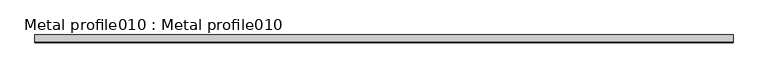
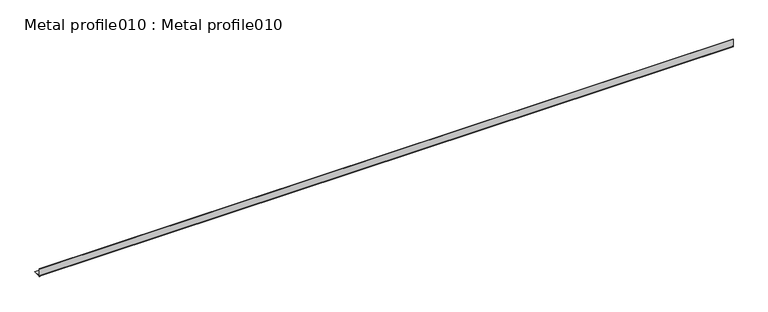
"""IFC4 building model written with IfcOpenShell, lengths in millimetres: proxy geometry, Metal profile010 : Metal profile010."""

import ifcopenshell
import ifcopenshell.guid

model = None  # the IFC model being written
_history = None  # IfcOwnerHistory: only IFC2X3 demands one
_inside = {}  # id of a spatial element -> (the spatial element, [elements in it])
_under = {}  # id of a project, library or spatial element -> (it, [spatial elements below it])
_declared = {}  # id of a project -> (the project, [libraries it declares])
_typed = {}  # id of a type object -> (the type object, [elements of that type])
_made_of = {}  # id of a material, layer set ... -> (it, [elements and type objects made of it])


def new_model(schema):
    """Start an empty IFC model of exactly this schema.

    Asked for "IFC4X3", IfcOpenShell would pick the latest addendum, in which some entities
    have other attributes; the version numbers below select the first issue.
    IFC2X3 requires an IfcOwnerHistory on every rooted entity: one is made here for all.
    """
    global model, _history
    if schema == "IFC4X3":
        model = ifcopenshell.file(schema_version=(4, 3, 0, 0))
    else:
        model = ifcopenshell.file(schema=schema)
    _inside.clear()
    _under.clear()
    _declared.clear()
    _typed.clear()
    _made_of.clear()
    _history = None
    if model.schema == "IFC2X3":
        org = make("IfcOrganization", Name="unknown")
        user = make(
            "IfcPersonAndOrganization",
            ThePerson=make("IfcPerson", FamilyName="unknown"),
            TheOrganization=org,
        )
        app = make(
            "IfcApplication",
            ApplicationDeveloper=org,
            Version="unknown",
            ApplicationFullName="unknown",
            ApplicationIdentifier="unknown",
        )
        _history = make(
            "IfcOwnerHistory",
            OwningUser=user,
            OwningApplication=app,
            ChangeAction="ADDED",
            CreationDate=0,
        )
    return model


def make(cls, **values):
    """One entity of the class cls with the attributes given. An attribute that is None is left unset."""
    return model.create_entity(
        cls, **{name: value for name, value in values.items() if value is not None}
    )


def rooted(cls, **values):
    """An entity with a GlobalId (a new one), such as an element, a storey or a relation."""
    return make(cls, GlobalId=ifcopenshell.guid.new(), OwnerHistory=_history, **values)


def si_unit(unit_type, name, prefix=None):
    """IfcSIUnit, for example si_unit("LENGTHUNIT", "METRE", prefix="MILLI")."""
    return make("IfcSIUnit", UnitType=unit_type, Prefix=prefix, Name=name)


def assignment(units):
    """IfcUnitAssignment: the units of a project."""
    return None if units is None else make("IfcUnitAssignment", Units=units)


def point(xyz):
    """IfcCartesianPoint."""
    return None if xyz is None else make("IfcCartesianPoint", Coordinates=xyz)


def direction(xyz):
    """IfcDirection."""
    return None if xyz is None else make("IfcDirection", DirectionRatios=xyz)


def frame(location, z_axis=None, x_axis=None):
    """IfcAxis2Placement3D, a coordinate frame: its origin and axes. An axis left out is left unset."""
    return make(
        "IfcAxis2Placement3D",
        Location=point(location),
        Axis=direction(z_axis),
        RefDirection=direction(x_axis),
    )


def frame_2d(location, x_axis=None):
    """IfcAxis2Placement2D, a coordinate frame in the plane: its origin and x axis."""
    return make(
        "IfcAxis2Placement2D", Location=point(location), RefDirection=direction(x_axis)
    )


def origin():
    """The frame at (0, 0, 0) with its axes left unset."""
    return frame((0.0, 0.0, 0.0))


def place(relative_to, where):
    """IfcLocalPlacement: puts the frame where relative to a parent placement (None: the world)."""
    return make(
        "IfcLocalPlacement", PlacementRelTo=relative_to, RelativePlacement=where
    )


def context(
    kind, dimensions, precision=None, world=None, true_north=None, identifier=None
):
    """IfcGeometricRepresentationContext, for example the 3D "Model" context."""
    return make(
        "IfcGeometricRepresentationContext",
        ContextIdentifier=identifier,
        ContextType=kind,
        CoordinateSpaceDimension=dimensions,
        Precision=precision,
        WorldCoordinateSystem=world,
        TrueNorth=true_north,
    )


def project(units=None, contexts=None):
    """IfcProject with its units and contexts."""
    return rooted(
        "IfcProject",
        Name="project",
        RepresentationContexts=contexts,
        UnitsInContext=assignment(units),
    )


def spatial(cls, under=None, at=None, **own):
    """A site, building, storey or space (cls), placed at a placement, below another one or the project."""
    s = rooted(cls, ObjectPlacement=at, **own)
    if under is not None:
        _under.setdefault(under.id(), (under, []))[1].append(s)
    return s


def polyline(points):
    """IfcPolyline through the points."""
    return make("IfcPolyline", Points=[point(p) for p in points])


def circle_curve(where, radius):
    """IfcCircle in the frame where."""
    return make("IfcCircle", Position=where, Radius=radius)


def trimmed(basis, trim1, trim2, sense, master):
    """IfcTrimmedCurve: the piece of a basis curve between two trims."""
    return make(
        "IfcTrimmedCurve",
        BasisCurve=basis,
        Trim1=trim1,
        Trim2=trim2,
        SenseAgreement=sense,
        MasterRepresentation=master,
    )


def segment(curve, same_sense, transition):
    """IfcCompositeCurveSegment."""
    return make(
        "IfcCompositeCurveSegment",
        Transition=transition,
        SameSense=same_sense,
        ParentCurve=curve,
    )


def composite_curve(segments, self_intersect=None):
    """IfcCompositeCurve: segments joined end to end."""
    return make("IfcCompositeCurve", Segments=segments, SelfIntersect=self_intersect)


def outline(outer, holes=None, kind="AREA"):
    """IfcArbitraryClosedProfileDef: a profile drawn as a closed curve; with holes, ...WithVoids."""
    if holes is None:
        return make("IfcArbitraryClosedProfileDef", ProfileType=kind, OuterCurve=outer)
    return make(
        "IfcArbitraryProfileDefWithVoids",
        ProfileType=kind,
        OuterCurve=outer,
        InnerCurves=holes,
    )


def extrude(swept, where, along, depth):
    """IfcExtrudedAreaSolid: the profile swept, set in the frame where, extruded along a direction by depth."""
    return make(
        "IfcExtrudedAreaSolid",
        SweptArea=swept,
        Position=where,
        ExtrudedDirection=direction(along),
        Depth=depth,
    )


def shape(context_of_items, identifier, shape_type, items):
    """IfcShapeRepresentation: the items that make up one representation, for example the "Body"."""
    return make(
        "IfcShapeRepresentation",
        ContextOfItems=context_of_items,
        RepresentationIdentifier=identifier,
        RepresentationType=shape_type,
        Items=items,
    )


def source(mapping_origin, context_of_items, identifier, shape_type, items):
    """IfcRepresentationMap: a shape defined once, which mapped items show again and again."""
    return make(
        "IfcRepresentationMap",
        MappingOrigin=mapping_origin,
        MappedRepresentation=shape(context_of_items, identifier, shape_type, items),
    )


def transform(
    local_origin,
    x_axis=None,
    y_axis=None,
    z_axis=None,
    scale=None,
    scale2=None,
    scale3=None,
    uniform=True,
):
    """IfcCartesianTransformationOperator3D, or its non-uniform kind. x_axis, y_axis, z_axis: its Axis1, 2, 3."""
    if uniform:
        return make(
            "IfcCartesianTransformationOperator3D",
            Axis1=direction(x_axis),
            Axis2=direction(y_axis),
            LocalOrigin=point(local_origin),
            Scale=scale,
            Axis3=direction(z_axis),
        )
    return make(
        "IfcCartesianTransformationOperator3DnonUniform",
        Axis1=direction(x_axis),
        Axis2=direction(y_axis),
        LocalOrigin=point(local_origin),
        Scale=scale,
        Axis3=direction(z_axis),
        Scale2=scale2,
        Scale3=scale3,
    )


def mapped(mapping_source, mapping_target):
    """IfcMappedItem: shows the shape of a source again, moved by a transform."""
    return make(
        "IfcMappedItem", MappingSource=mapping_source, MappingTarget=mapping_target
    )


def made_of(thing, what):
    """Note that an element or type object is made of a material, layer set ...; save() writes the relation."""
    if what is not None:
        _made_of.setdefault(what.id(), (what, []))[1].append(thing)
    return thing


def element(
    cls,
    number,
    at=None,
    inside=None,
    cuts=None,
    type_object=None,
    material=None,
    context=None,
    identifier="Body",
    shape_type=None,
    held_by="IfcProductDefinitionShape",
    body=None,
    shapes=None,
    **own,
):
    """One element of the class cls, such as IfcWall. Its Tag is "e" and its number.

    at: its placement. inside: the storey or other place that contains it. cuts: it is an
    opening in that element (IfcRelVoidsElement). A single representation is given by context,
    identifier, shape_type and body (its items); several are given by shapes. held_by: the class
    of the entity that holds the representations. save() writes the other relations.
    """
    e = rooted(cls, Tag="e%d" % number, ObjectPlacement=at, **own)
    if body is not None:
        shapes = [shape(context, identifier, shape_type, body)]
    if shapes is not None:
        e.Representation = make(held_by, Representations=shapes)
    if inside is not None:
        _inside.setdefault(inside.id(), (inside, []))[1].append(e)
    if cuts is not None:
        rooted(
            "IfcRelVoidsElement", RelatingBuildingElement=cuts, RelatedOpeningElement=e
        )
    if type_object is not None:
        _typed.setdefault(type_object.id(), (type_object, []))[1].append(e)
    return made_of(e, material)


def aggregate(whole, parts):
    """IfcRelAggregates: a whole, such as a stair, and the parts it consists of."""
    return rooted("IfcRelAggregates", RelatingObject=whole, RelatedObjects=parts)


def save(model, path):
    """Write the relations noted so far, then the file.

    IfcRelAggregates (storeys below a building ...), IfcRelContainedInSpatialStructure (elements
    in a storey), IfcRelDefinesByType, IfcRelAssociatesMaterial and IfcRelDeclares: one each for
    every whole, place, type object, material and project.
    """
    for whole, parts in _under.values():
        aggregate(whole, parts)
    for where, things in _inside.values():
        rooted(
            "IfcRelContainedInSpatialStructure",
            RelatedElements=things,
            RelatingStructure=where,
        )
    for kind, things in _typed.values():
        rooted("IfcRelDefinesByType", RelatedObjects=things, RelatingType=kind)
    for what, things in _made_of.values():
        rooted("IfcRelAssociatesMaterial", RelatedObjects=things, RelatingMaterial=what)
    for by, libraries in _declared.values():
        rooted("IfcRelDeclares", RelatingContext=by, RelatedDefinitions=libraries)
    model.write(path)


def metal_profile010_metal_profile010_d71006e5(model_context):
    return source(origin(), model_context, "Body", "SweptSolid", [
        extrude(outline(composite_curve([segment(polyline([(10263.4300834, 42913.2541839), (10263.4300834, 42892.101), (10284.5832673, 42892.101), (10284.5832673, 42890.821), (10263.6803576, 42890.821)]), True, "CONTINUOUS"), segment(trimmed(circle_curve(frame_2d((10262.7900834, 42891.461)), 1.0964434), [point((10263.6803576, 42890.821))], [point((10262.1500834, 42892.3512742))], False, "CARTESIAN"), True, "CONTINUOUS"), segment(polyline([(10262.1500834, 42892.3512742), (10262.1500834, 42913.2541839), (10263.4300834, 42913.2541839)]), True, "CONTINUOUS")], self_intersect=False)), frame((3694.2883192, 0.0, 0.0), z_axis=(1.0, 0.0, 0.0), x_axis=(0.0, 1.0, 0.0)), (0.0, 0.0, 1.0), 2000.0),
    ])


if __name__ == "__main__":
    model = new_model("IFC4")
    model_context = context("Model", 3, world=origin())
    ifc_project = project(units=[si_unit("LENGTHUNIT", "METRE", prefix="MILLI")], contexts=[model_context])
    site = spatial("IfcSite", under=ifc_project)
    building = spatial("IfcBuilding", under=site)
    placement = place(None, origin())
    metal_profile010_metal_profile010_shape = metal_profile010_metal_profile010_d71006e5(model_context)
    element("IfcBuildingElementProxy", 1, Name="Metal profile010 : Metal profile010", ObjectType="Metal profile010 : Metal profile010", at=placement, inside=building, context=model_context, shape_type="MappedRepresentation", body=[
        mapped(metal_profile010_metal_profile010_shape, transform((0.0, 0.0, 0.0), x_axis=(1.0, 0.0, 0.0), y_axis=(0.0, 1.0, 0.0), z_axis=(0.0, 0.0, 1.0))),
    ])
    save(model, "model.ifc")

# Revit data of these elements
# Type "Metal profile010 : Metal profile010"
#   NameOverride = "Metal profile010"
# Element 1 (IfcBuildingElementProxy, "Metal profile010 : Metal profile010")
#   Materials on its faces: "CORNER BEAD"
# Materials
#   "CORNER BEAD": class "Unassigned", colour RGB 253 236 176, transparency 0, Cost = 0
